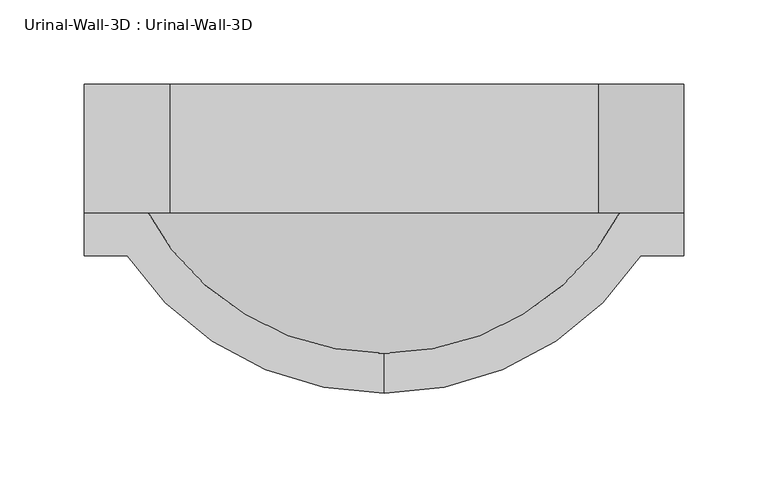
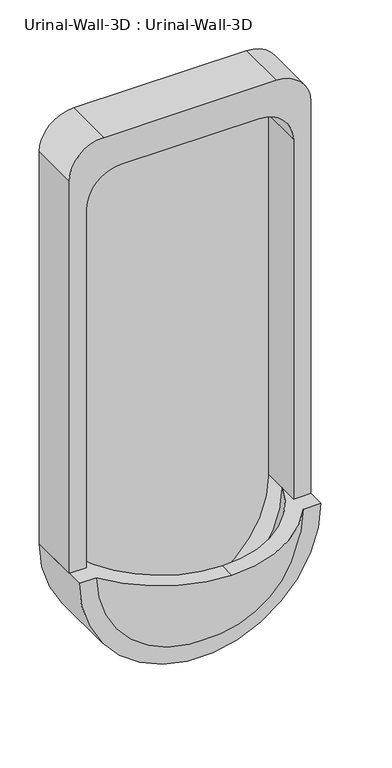
"""IFC4 building model written with IfcOpenShell, lengths in millimetres: flow terminal geometry, Urinal-Wall-3D : Urinal-Wall-3D."""

import ifcopenshell
import ifcopenshell.guid

model = None  # the IFC model being written
_history = None  # IfcOwnerHistory: only IFC2X3 demands one
_inside = {}  # id of a spatial element -> (the spatial element, [elements in it])
_under = {}  # id of a project, library or spatial element -> (it, [spatial elements below it])
_declared = {}  # id of a project -> (the project, [libraries it declares])
_typed = {}  # id of a type object -> (the type object, [elements of that type])
_made_of = {}  # id of a material, layer set ... -> (it, [elements and type objects made of it])


def new_model(schema):
    """Start an empty IFC model of exactly this schema.

    Asked for "IFC4X3", IfcOpenShell would pick the latest addendum, in which some entities
    have other attributes; the version numbers below select the first issue.
    IFC2X3 requires an IfcOwnerHistory on every rooted entity: one is made here for all.
    """
    global model, _history
    if schema == "IFC4X3":
        model = ifcopenshell.file(schema_version=(4, 3, 0, 0))
    else:
        model = ifcopenshell.file(schema=schema)
    _inside.clear()
    _under.clear()
    _declared.clear()
    _typed.clear()
    _made_of.clear()
    _history = None
    if model.schema == "IFC2X3":
        org = make("IfcOrganization", Name="unknown")
        user = make(
            "IfcPersonAndOrganization",
            ThePerson=make("IfcPerson", FamilyName="unknown"),
            TheOrganization=org,
        )
        app = make(
            "IfcApplication",
            ApplicationDeveloper=org,
            Version="unknown",
            ApplicationFullName="unknown",
            ApplicationIdentifier="unknown",
        )
        _history = make(
            "IfcOwnerHistory",
            OwningUser=user,
            OwningApplication=app,
            ChangeAction="ADDED",
            CreationDate=0,
        )
    return model


def make(cls, **values):
    """One entity of the class cls with the attributes given. An attribute that is None is left unset."""
    return model.create_entity(
        cls, **{name: value for name, value in values.items() if value is not None}
    )


def rooted(cls, **values):
    """An entity with a GlobalId (a new one), such as an element, a storey or a relation."""
    return make(cls, GlobalId=ifcopenshell.guid.new(), OwnerHistory=_history, **values)


def si_unit(unit_type, name, prefix=None):
    """IfcSIUnit, for example si_unit("LENGTHUNIT", "METRE", prefix="MILLI")."""
    return make("IfcSIUnit", UnitType=unit_type, Prefix=prefix, Name=name)


def assignment(units):
    """IfcUnitAssignment: the units of a project."""
    return None if units is None else make("IfcUnitAssignment", Units=units)


def point(xyz):
    """IfcCartesianPoint."""
    return None if xyz is None else make("IfcCartesianPoint", Coordinates=xyz)


def direction(xyz):
    """IfcDirection."""
    return None if xyz is None else make("IfcDirection", DirectionRatios=xyz)


def frame(location, z_axis=None, x_axis=None):
    """IfcAxis2Placement3D, a coordinate frame: its origin and axes. An axis left out is left unset."""
    return make(
        "IfcAxis2Placement3D",
        Location=point(location),
        Axis=direction(z_axis),
        RefDirection=direction(x_axis),
    )


def frame_2d(location, x_axis=None):
    """IfcAxis2Placement2D, a coordinate frame in the plane: its origin and x axis."""
    return make(
        "IfcAxis2Placement2D", Location=point(location), RefDirection=direction(x_axis)
    )


def origin():
    """The frame at (0, 0, 0) with its axes left unset."""
    return frame((0.0, 0.0, 0.0))


def place(relative_to, where):
    """IfcLocalPlacement: puts the frame where relative to a parent placement (None: the world)."""
    return make(
        "IfcLocalPlacement", PlacementRelTo=relative_to, RelativePlacement=where
    )


def context(
    kind, dimensions, precision=None, world=None, true_north=None, identifier=None
):
    """IfcGeometricRepresentationContext, for example the 3D "Model" context."""
    return make(
        "IfcGeometricRepresentationContext",
        ContextIdentifier=identifier,
        ContextType=kind,
        CoordinateSpaceDimension=dimensions,
        Precision=precision,
        WorldCoordinateSystem=world,
        TrueNorth=true_north,
    )


def project(units=None, contexts=None):
    """IfcProject with its units and contexts."""
    return rooted(
        "IfcProject",
        Name="project",
        RepresentationContexts=contexts,
        UnitsInContext=assignment(units),
    )


def spatial(cls, under=None, at=None, **own):
    """A site, building, storey or space (cls), placed at a placement, below another one or the project."""
    s = rooted(cls, ObjectPlacement=at, **own)
    if under is not None:
        _under.setdefault(under.id(), (under, []))[1].append(s)
    return s


def polyline(points):
    """IfcPolyline through the points."""
    return make("IfcPolyline", Points=[point(p) for p in points])


def circle_curve(where, radius):
    """IfcCircle in the frame where."""
    return make("IfcCircle", Position=where, Radius=radius)


def ellipse_curve(where, semi_axis1, semi_axis2):
    """IfcEllipse in the frame where."""
    return make(
        "IfcEllipse", Position=where, SemiAxis1=semi_axis1, SemiAxis2=semi_axis2
    )


def trimmed(basis, trim1, trim2, sense, master):
    """IfcTrimmedCurve: the piece of a basis curve between two trims."""
    return make(
        "IfcTrimmedCurve",
        BasisCurve=basis,
        Trim1=trim1,
        Trim2=trim2,
        SenseAgreement=sense,
        MasterRepresentation=master,
    )


def segment(curve, same_sense, transition):
    """IfcCompositeCurveSegment."""
    return make(
        "IfcCompositeCurveSegment",
        Transition=transition,
        SameSense=same_sense,
        ParentCurve=curve,
    )


def composite_curve(segments, self_intersect=None):
    """IfcCompositeCurve: segments joined end to end."""
    return make("IfcCompositeCurve", Segments=segments, SelfIntersect=self_intersect)


def outline(outer, holes=None, kind="AREA"):
    """IfcArbitraryClosedProfileDef: a profile drawn as a closed curve; with holes, ...WithVoids."""
    if holes is None:
        return make("IfcArbitraryClosedProfileDef", ProfileType=kind, OuterCurve=outer)
    return make(
        "IfcArbitraryProfileDefWithVoids",
        ProfileType=kind,
        OuterCurve=outer,
        InnerCurves=holes,
    )


def extrude(swept, where, along, depth):
    """IfcExtrudedAreaSolid: the profile swept, set in the frame where, extruded along a direction by depth."""
    return make(
        "IfcExtrudedAreaSolid",
        SweptArea=swept,
        Position=where,
        ExtrudedDirection=direction(along),
        Depth=depth,
    )


def shape(context_of_items, identifier, shape_type, items):
    """IfcShapeRepresentation: the items that make up one representation, for example the "Body"."""
    return make(
        "IfcShapeRepresentation",
        ContextOfItems=context_of_items,
        RepresentationIdentifier=identifier,
        RepresentationType=shape_type,
        Items=items,
    )


def source(mapping_origin, context_of_items, identifier, shape_type, items):
    """IfcRepresentationMap: a shape defined once, which mapped items show again and again."""
    return make(
        "IfcRepresentationMap",
        MappingOrigin=mapping_origin,
        MappedRepresentation=shape(context_of_items, identifier, shape_type, items),
    )


def transform(
    local_origin,
    x_axis=None,
    y_axis=None,
    z_axis=None,
    scale=None,
    scale2=None,
    scale3=None,
    uniform=True,
):
    """IfcCartesianTransformationOperator3D, or its non-uniform kind. x_axis, y_axis, z_axis: its Axis1, 2, 3."""
    if uniform:
        return make(
            "IfcCartesianTransformationOperator3D",
            Axis1=direction(x_axis),
            Axis2=direction(y_axis),
            LocalOrigin=point(local_origin),
            Scale=scale,
            Axis3=direction(z_axis),
        )
    return make(
        "IfcCartesianTransformationOperator3DnonUniform",
        Axis1=direction(x_axis),
        Axis2=direction(y_axis),
        LocalOrigin=point(local_origin),
        Scale=scale,
        Axis3=direction(z_axis),
        Scale2=scale2,
        Scale3=scale3,
    )


def mapped(mapping_source, mapping_target):
    """IfcMappedItem: shows the shape of a source again, moved by a transform."""
    return make(
        "IfcMappedItem", MappingSource=mapping_source, MappingTarget=mapping_target
    )


def made_of(thing, what):
    """Note that an element or type object is made of a material, layer set ...; save() writes the relation."""
    if what is not None:
        _made_of.setdefault(what.id(), (what, []))[1].append(thing)
    return thing


def element(
    cls,
    number,
    at=None,
    inside=None,
    cuts=None,
    type_object=None,
    material=None,
    context=None,
    identifier="Body",
    shape_type=None,
    held_by="IfcProductDefinitionShape",
    body=None,
    shapes=None,
    **own,
):
    """One element of the class cls, such as IfcWall. Its Tag is "e" and its number.

    at: its placement. inside: the storey or other place that contains it. cuts: it is an
    opening in that element (IfcRelVoidsElement). A single representation is given by context,
    identifier, shape_type and body (its items); several are given by shapes. held_by: the class
    of the entity that holds the representations. save() writes the other relations.
    """
    e = rooted(cls, Tag="e%d" % number, ObjectPlacement=at, **own)
    if body is not None:
        shapes = [shape(context, identifier, shape_type, body)]
    if shapes is not None:
        e.Representation = make(held_by, Representations=shapes)
    if inside is not None:
        _inside.setdefault(inside.id(), (inside, []))[1].append(e)
    if cuts is not None:
        rooted(
            "IfcRelVoidsElement", RelatingBuildingElement=cuts, RelatedOpeningElement=e
        )
    if type_object is not None:
        _typed.setdefault(type_object.id(), (type_object, []))[1].append(e)
    return made_of(e, material)


def aggregate(whole, parts):
    """IfcRelAggregates: a whole, such as a stair, and the parts it consists of."""
    return rooted("IfcRelAggregates", RelatingObject=whole, RelatedObjects=parts)


def save(model, path):
    """Write the relations noted so far, then the file.

    IfcRelAggregates (storeys below a building ...), IfcRelContainedInSpatialStructure (elements
    in a storey), IfcRelDefinesByType, IfcRelAssociatesMaterial and IfcRelDeclares: one each for
    every whole, place, type object, material and project.
    """
    for whole, parts in _under.values():
        aggregate(whole, parts)
    for where, things in _inside.values():
        rooted(
            "IfcRelContainedInSpatialStructure",
            RelatedElements=things,
            RelatingStructure=where,
        )
    for kind, things in _typed.values():
        rooted("IfcRelDefinesByType", RelatedObjects=things, RelatingType=kind)
    for what, things in _made_of.values():
        rooted("IfcRelAssociatesMaterial", RelatedObjects=things, RelatingMaterial=what)
    for by, libraries in _declared.values():
        rooted("IfcRelDeclares", RelatingContext=by, RelatedDefinitions=libraries)
    model.write(path)


def plane_surface(at):
    """IfcPlane: the flat surface through the origin of the frame at, square to its z axis."""
    return make("IfcPlane", Position=at)


def cylinder_surface(at, radius):
    """IfcCylindricalSurface: all points at the distance radius from the z axis of the frame at."""
    return make("IfcCylindricalSurface", Position=at, Radius=radius)


def revolved_surface(curve, axis_point, axis_direction):
    """IfcSurfaceOfRevolution: the curve turned about the line through axis_point along axis_direction."""
    return make(
        "IfcSurfaceOfRevolution",
        SweptCurve=make("IfcArbitraryOpenProfileDef", ProfileType="CURVE", Curve=curve),
        AxisPosition=make("IfcAxis1Placement", Location=point(axis_point), Axis=direction(axis_direction)),
    )


def advanced_brep(points, edges, surfaces, faces):
    """IfcAdvancedBrep: a solid bounded by faces that lie on surfaces and meet in shared edges.

    An edge is (start, end): straight between two places in points (the first is 0);
    or (start, end, curve); or (start, end, curve, False) where it runs against its curve.
    A face is (place in surfaces, loops), or (place, loops, False) where it looks against
    its surface's normal. A loop lists edges by number (the first is 1), with a minus sign
    where the edge is run from its end to its start. The first loop is the outer one.
    """
    corners = [point(p) for p in points]
    vertices = [make("IfcVertexPoint", VertexGeometry=c) for c in corners]
    made = []
    for start, end, *more in edges:
        made.append(
            make(
                "IfcEdgeCurve",
                EdgeStart=vertices[start],
                EdgeEnd=vertices[end],
                EdgeGeometry=more[0] if more else make("IfcPolyline", Points=[corners[start], corners[end]]),
                SameSense=more[1] if len(more) > 1 else True,
            )
        )
    hull = []
    for where, loops, *sense in faces:
        bounds = []
        for j, loop in enumerate(loops):
            ring = [make("IfcOrientedEdge", EdgeElement=made[abs(k) - 1], Orientation=k > 0) for k in loop]
            bounds.append(
                make(
                    "IfcFaceOuterBound" if j == 0 else "IfcFaceBound",
                    Bound=make("IfcEdgeLoop", EdgeList=ring),
                    Orientation=True,
                )
            )
        hull.append(make("IfcAdvancedFace", Bounds=bounds, FaceSurface=surfaces[where], SameSense=sense[0] if sense else True))
    return make("IfcAdvancedBrep", Outer=make("IfcClosedShell", CfsFaces=hull))


def urinal_wall_3d_urinal_wall_3d_87f6c982(model_context):
    return source(origin(), model_context, "Body", "SolidModel", [
        extrude(outline(composite_curve([segment(polyline([(609.6, 43.3254001), (609.6, 68.7254001), (1219.2, 68.7254001)]), True, "CONTINUOUS"), segment(trimmed(circle_curve(frame_2d((1219.2, 17.9254001)), 50.8), [point((1219.2, 68.7254001))], [point((1270.0, 17.9254001))], False, "CARTESIAN"), True, "CONTINUOUS"), segment(polyline([(1270.0, 17.9254001), (1270.0, -236.0745999)]), True, "CONTINUOUS"), segment(trimmed(circle_curve(frame_2d((1219.2, -236.0745999)), 50.8), [point((1270.0, -236.0745999))], [point((1219.2, -286.8745999))], False, "CARTESIAN"), True, "CONTINUOUS"), segment(polyline([(1219.2, -286.8745999), (609.6, -286.8745999), (609.6, -261.4745999), (1168.4, -261.4745999)]), True, "CONTINUOUS"), segment(trimmed(circle_curve(frame_2d((1168.4, -210.6745999)), 50.8), [point((1168.4, -261.4745999))], [point((1219.2, -210.6745999))], True, "CARTESIAN"), True, "CONTINUOUS"), segment(polyline([(1219.2, -210.6745999), (1219.2, -7.4745999)]), True, "CONTINUOUS"), segment(trimmed(circle_curve(frame_2d((1168.4, -7.4745999)), 50.8), [point((1219.2, -7.4745999))], [point((1168.4, 43.3254001))], True, "CARTESIAN"), True, "CONTINUOUS"), segment(polyline([(1168.4, 43.3254001), (609.6, 43.3254001)]), True, "CONTINUOUS")], self_intersect=False)), frame((0.0, -274.6375, 0.0), z_axis=(0.0, 1.0, 0.0), x_axis=(0.0, 0.0, 1.0)), (0.0, 0.0, 1.0), 76.2),
        extrude(outline(composite_curve([segment(trimmed(circle_curve(frame_2d((1168.4, -7.4745999)), 50.8), [point((1168.4, 43.3254001))], [point((1219.2, -7.4745999))], False, "CARTESIAN"), True, "CONTINUOUS"), segment(polyline([(1219.2, -7.4745999), (1219.2, -210.6745999)]), True, "CONTINUOUS"), segment(trimmed(circle_curve(frame_2d((1168.4, -210.6745999)), 50.8), [point((1219.2, -210.6745999))], [point((1168.4, -261.4745999))], False, "CARTESIAN"), True, "CONTINUOUS"), segment(polyline([(1168.4, -261.4745999), (609.6, -261.4745999)]), True, "CONTINUOUS"), segment(trimmed(circle_curve(frame_2d((609.6, -109.0745999)), 152.4), [point((609.6, -261.4745999))], [point((609.6, 43.3254001))], False, "CARTESIAN"), True, "CONTINUOUS"), segment(polyline([(609.6, 43.3254001), (1168.4, 43.3254001)]), True, "CONTINUOUS")], self_intersect=False)), frame((0.0, -211.1375, 0.0), z_axis=(0.0, 1.0, 0.0), x_axis=(0.0, 0.0, 1.0)), (0.0, 0.0, 1.0), 12.7),
        advanced_brep(
        [(-109.0745999, -381.5995048, 609.6), (43.3254001, -300.0375, 609.6), (68.7254001, -300.0375, 609.6), (68.7254001, -198.4375, 609.6), (43.3254001, -198.4375, 609.6), (43.3254001, -245.3081063, 609.6), (-109.0745999, -357.8822043, 609.6), (-261.4745999, -245.3081063, 609.6), (-261.4745999, -198.4375, 609.6), (-286.8745999, -198.4375, 609.6), (-286.8745999, -300.0375, 609.6), (-261.4745999, -300.0375, 609.6)],
        [
            (0, 1, circle_curve(frame((-109.0745999, -198.4375, 609.6), z_axis=(0.0, 0.0, 1.0), x_axis=(1.0, 0.0, 0.0)), 183.1620048)),
            (1, 2),
            (2, 3),
            (3, 4),
            (4, 5),
            (5, 6, circle_curve(frame((-109.0745999, -198.4375, 609.6), z_axis=(0.0, 0.0, -1.0), x_axis=(1.0, 0.0, 0.0)), 159.4447043)),
            (6, 0),
            (6, 7, circle_curve(frame((-109.0745999, -198.4375, 609.6), z_axis=(0.0, 0.0, -1.0), x_axis=(-1.0, 0.0, 0.0)), 159.4447043)),
            (7, 8),
            (8, 9),
            (9, 10),
            (10, 11),
            (11, 0, circle_curve(frame((-109.0745999, -198.4375, 609.6), z_axis=(0.0, 0.0, 1.0), x_axis=(-1.0, 0.0, 0.0)), 183.1620048)),
            (5, 7, circle_curve(frame((-109.0745999, -245.3081063, 609.6), z_axis=(0.0, 1.0, 0.0), x_axis=(1.0, 0.0, 0.0)), 152.4)),
            (4, 8, circle_curve(frame((-109.0745999, -198.4375, 609.6), z_axis=(0.0, 1.0, 0.0), x_axis=(1.0, 0.0, 0.0)), 152.4)),
            (3, 9, circle_curve(frame((-109.0745999, -198.4375, 609.6), z_axis=(0.0, 1.0, 0.0), x_axis=(1.0, 0.0, 0.0)), 177.8)),
            (2, 10, circle_curve(frame((-109.0745999, -300.0375, 609.6), z_axis=(0.0, 1.0, 0.0), x_axis=(1.0, 0.0, 0.0)), 177.8)),
            (1, 11, circle_curve(frame((-109.0745999, -300.0375, 609.6), z_axis=(0.0, 1.0, 0.0), x_axis=(1.0, 0.0, 0.0)), 152.4)),
        ],
        [
            plane_surface(frame((-109.0745999, -487.6479173, 609.6), z_axis=(0.0, 0.0, 1.0), x_axis=(1.0, 0.0, 0.0))),
            plane_surface(frame((-109.0745999, -487.6479173, 609.6), z_axis=(0.0, 0.0, 1.0), x_axis=(-1.0, 0.0, 0.0))),
            revolved_surface(trimmed(ellipse_curve(frame((-109.0745999, -198.4375, 609.6), z_axis=(0.0, 0.0, 1.0), x_axis=(1.0, 0.0, 0.0)), 159.4447043, 159.4447043), [point((-109.0745999, -357.8822043, 609.6))], [point((43.3254001, -245.3081063, 609.6))], True, "CARTESIAN"), (-109.0745999, -487.6479173, 609.6), (0.0, -1.0, 0.0)),
            revolved_surface(polyline([(43.32540010000001, -245.3081063, 609.6), (43.32540010000001, -198.4375, 609.6)]), (-109.0745999, -487.6479173, 609.6), (0.0, -1.0, 0.0)),
            plane_surface(frame((-109.0745999, -198.4375, 609.6), z_axis=(0.0, 1.0, 0.0), x_axis=(1.0, 0.0, 0.0))),
            cylinder_surface(frame((-109.0745999, -487.6479173, 609.6), z_axis=(0.0, -1.0, 0.0), x_axis=(1.0, 0.0, 0.0)), 177.8),
            plane_surface(frame((-109.0745999, -300.0375, 609.6), z_axis=(0.0, -1.0, 0.0), x_axis=(1.0, 0.0, 0.0))),
            revolved_surface(trimmed(ellipse_curve(frame((-109.0745999, -198.4375, 609.6), z_axis=(0.0, 0.0, -1.0), x_axis=(1.0, 0.0, 0.0)), 183.1620048, 183.1620048), [point((43.3254001, -300.0375, 609.6))], [point((-109.0745999, -381.5995048, 609.6))], True, "CARTESIAN"), (-109.0745999, -487.6479173, 609.6), (0.0, -1.0, 0.0)),
        ],
        [
            (0, [[1, 2, 3, 4, 5, 6, 7]]),
            (1, [[-7, 8, 9, 10, 11, 12, 13]]),
            (2, [[-8, -6, 14]]),
            (3, [[-9, -14, -5, 15]]),
            (4, [[-10, -15, -4, 16]]),
            (5, [[-11, -16, -3, 17]]),
            (6, [[-12, -17, -2, 18]]),
            (7, [[-13, -18, -1]]),
        ],
    ),
    ])


if __name__ == "__main__":
    model = new_model("IFC4")
    model_context = context("Model", 3, world=origin())
    ifc_project = project(units=[si_unit("LENGTHUNIT", "METRE", prefix="MILLI")], contexts=[model_context])
    site = spatial("IfcSite", under=ifc_project)
    building = spatial("IfcBuilding", under=site)
    placement = place(None, origin())
    urinal_wall_3d_urinal_wall_3d_shape = urinal_wall_3d_urinal_wall_3d_87f6c982(model_context)
    element("IfcFlowTerminal", 1, ObjectType="Urinal-Wall-3D : Urinal-Wall-3D", at=placement, inside=building, context=model_context, shape_type="MappedRepresentation", body=[
        mapped(urinal_wall_3d_urinal_wall_3d_shape, transform((0.0, 0.0, 0.0), x_axis=(1.0, 0.0, 0.0), y_axis=(0.0, 1.0, 0.0), z_axis=(0.0, 0.0, 1.0))),
    ])
    save(model, "model.ifc")

# Revit data of these elements
# Type "Urinal-Wall-3D : Urinal-Wall-3D"
#   Assembly Code = "D2010210"
#   Bowl Height = 2' - 0"
#   Urinal Material = Porcelain - Ivory
#   Default Elevation = 0
# Materials
#   "Porcelain - Ivory": class "Unassigned", colour RGB 247 247 239, transparency 0
